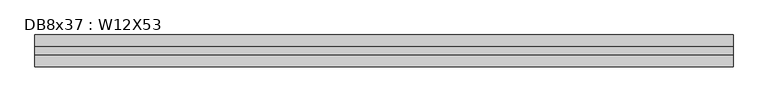
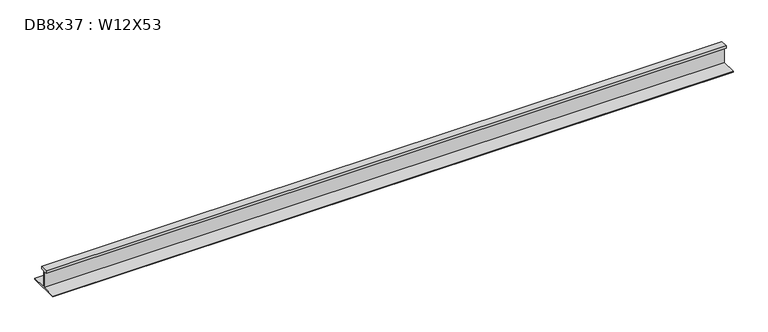
"""IFC4 building model written with IfcOpenShell, lengths in millimetres: beam geometry, DB8x37 : W12X53."""

from ifc_helpers import new_model, si_unit, frame, origin, place, context, project, spatial, polyline, outline, extrude, source, transform, mapped, element, save


def db8x37_w12x53_0f4ab858(model_context):
    return source(origin(), model_context, "Body", "SweptSolid", [
        extrude(outline(polyline([(38.1, 145.415), (38.1, 120.015), (2.921, 120.015), (2.921, -48.4505), (152.4, -48.4505), (152.4, -58.1025), (-152.4, -58.1025), (-152.4, -48.4505), (-2.921, -48.4505), (-2.921, 120.015), (-38.1, 120.015), (-38.1, 145.415), (38.1, 145.415)])), frame((-3338.83, 0.0, 0.0), z_axis=(1.0, 0.0, 0.0), x_axis=(0.0, 1.0, 0.0)), (0.0, 0.0, 1.0), 6707.759),
    ])


if __name__ == "__main__":
    model = new_model("IFC4")
    model_context = context("Model", 3, world=origin())
    ifc_project = project(units=[si_unit("LENGTHUNIT", "METRE", prefix="MILLI")], contexts=[model_context])
    site = spatial("IfcSite", under=ifc_project)
    building = spatial("IfcBuilding", under=site)
    placement = place(None, origin())
    db8x37_w12x53_shape = db8x37_w12x53_0f4ab858(model_context)
    element("IfcBeam", 1, ObjectType="DB8x37 : W12X53", at=placement, inside=building, context=model_context, shape_type="MappedRepresentation", body=[
        mapped(db8x37_w12x53_shape, transform((0.0, 0.0, 0.0), x_axis=(1.0, 0.0, 0.0), y_axis=(0.0, 1.0, 0.0), z_axis=(0.0, 0.0, 1.0))),
    ])
    save(model, "model.ifc")

# Revit data of these elements
# Type "DB8x37 : W12X53"
#   Assembly Code = "B10"
#   W = 53
#   Length [instance default] = 5' - 0"
#   bf = 0' - 10"
#   d = 1' - 0.1"
#   k = 0' - 1 3/8"
#   k2 = 0' - 0.8"
#   tf = 0' - 0.575"
#   tw = 0' - 0.345"
#   A = 0.108333 SF
#   Structural Material [instance default] = Steel ASTM A992
# Element 1 (IfcBeam, "DB8x37 : W12X53")
#   Materials on its faces: "Steel ASTM A992"
# Materials
#   "Steel ASTM A992": class "Metal", colour RGB 199 199 199, transparency 0, Description = "Structural steel 50ksi", Cost = 0
